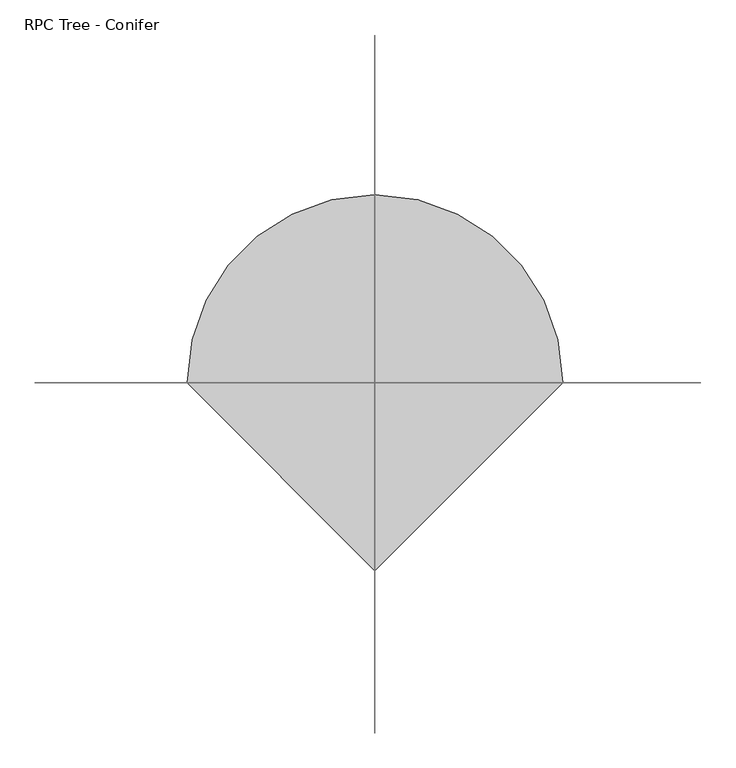
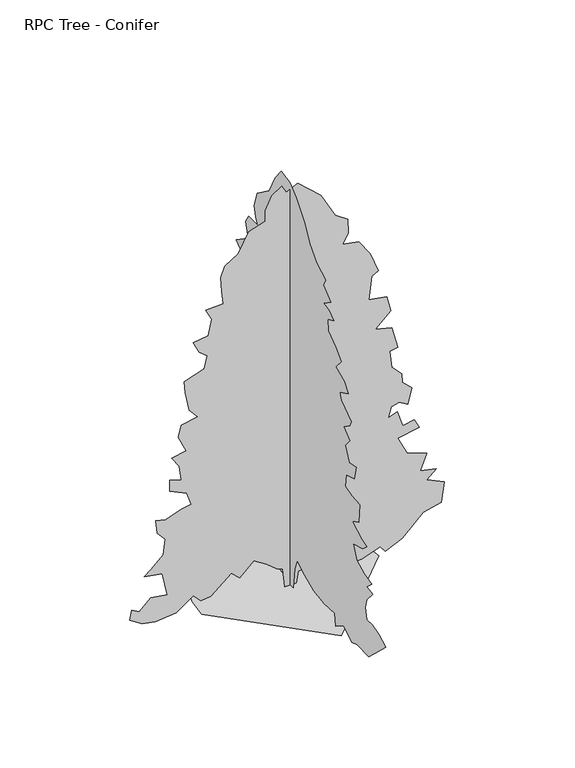
"""IFC4 building model written with IfcOpenShell, lengths in millimetres: geographic element geometry, RPC Tree - Conifer : Colorado Spruce - 13'."""

from ifc_helpers import new_model, si_unit, origin, place, context, project, spatial, triangles, source, transform, mapped, element, save


def rpc_tree_conifer_d3253eb6(model_context):
    return source(origin(), model_context, "Body", "Tessellation", [
        triangles([(0.1966733, -49.3561489, 3.58e-05), (0.1966807, -76.1744156, 207.8417467), (0.196685, -109.6973104, 301.7045676), (0.1966884, -230.379379, 234.6600225), (0.1966932, -377.8792239, 174.3188474), (0.1966999, -545.4937022, 147.5005898), (0.1967076, -713.5737408, 154.6348927), (0.196705, -733.2223234, 40.2275228), (0.1967129, -853.9046373, 120.682323), (0.196716, -981.9569956, 35.9934516), (0.1967211, -1075.1551586, 67.0457895), (0.196729, -1256.1798649, 60.3411615), (0.1967353, -1343.3377716, 140.7959572), (0.1967491, -1531.0664291, 321.8186923), (0.1967456, -1417.0879211, 375.4547353), (0.1967421, -1316.5197865, 408.9791061), (0.1967377, -1222.8412022, 401.1533847), (0.19674, -1202.5413511, 509.5473135), (0.196744, -1229.359409, 603.4116059), (0.1967514, -1323.2237377, 710.6836555), (0.1967478, -1229.359409, 730.7978348), (0.1967531, -1303.1095585, 797.8441057), (0.196749, -1189.1335939, 831.3659695), (0.1967454, -1068.45128, 891.7084345), (0.1967463, -1006.4049946, 1015.8652456), (0.1967546, -1162.3155361, 1059.3228401), (0.1967594, -1229.359409, 1119.6627617), (0.1967561, -1142.2014296, 1139.7769409), (0.1967521, -994.7010578, 1226.9373184), (0.1967585, -1101.9731438, 1280.5734341), (0.1967642, -1110.6508118, 1457.1305351), (0.1967592, -987.9947084, 1475.0058975), (0.1967552, -880.7226225, 1501.8238827), (0.1967595, -896.547456, 1623.9847401), (0.1967665, -1027.1927519, 1660.8127247), (0.1967716, -1055.0409794, 1790.1206749), (0.1967662, -947.7689661, 1770.0064957), (0.1967671, -880.024264, 1900.4932983), (0.1967731, -954.4728447, 1991.2570896), (0.1967713, -860.6085159, 2071.7111904), (0.1967775, -954.4728447, 2138.7573887), (0.1967803, -981.2908298, 2192.3935043), (0.196776, -813.6763515, 2299.6680611), (0.1967771, -793.562245, 2366.7117886), (0.1967851, -927.6547869, 2433.7581322), (0.196785, -867.3123945, 2520.9283928), (0.1967808, -733.2223234, 2581.2558151), (0.1967877, -820.3802301, 2681.8267113), (0.1967861, -726.515974, 2768.9745895), (0.1967833, -605.8360946, 2856.1474663), (0.1967862, -599.1297452, 2963.42929), (0.1967921, -699.6979162, 3010.3589836), (0.1967904, -625.9502375, 3064.0001862), (0.1967871, -538.7898236, 3084.1091331), (0.1967946, -652.7682226, 3164.5460838), (0.196792, -532.085945, 3258.4301788), (0.1967955, -565.6078451, 3325.4691101), (0.1967916, -424.8113883, 3405.9304779), (0.1967901, -310.832953, 3526.610321), (0.1967913, -235.627587, 3681.4162788), (0.1967901, -96.2880544, 3848.4313751), (0.1967879, 10.9852091, 3935.5795441), (0.1967827, 145.0765916, 3962.4), (0.1967749, 238.9406479, 3841.7201569), (0.1967651, 332.804468, 3654.0013824), (0.1967522, 527.2369314, 3513.1875938), (0.1967452, 580.8729744, 3359.0007843), (0.1967436, 554.0549529, 3265.1166893), (0.1967433, 520.5330528, 3204.7889763), (0.1967367, 668.0334246, 3204.7889763), (0.1967322, 714.9655163, 3124.3276085), (0.1967298, 674.7373032, 2983.5385277), (0.1967176, 862.465888, 2856.1474663), (0.1967187, 802.1234957, 2802.5065544), (0.1967143, 835.6479029, 2701.9356583), (0.1967057, 942.9199162, 2574.5445969), (0.1967072, 795.4196171, 2406.9400017), (0.1966989, 950.7208935, 2358.4253757), (0.1966939, 1036.7842449, 2319.782095), (0.1966878, 976.4418526, 2024.779026), (0.1966811, 1077.0125307, 1951.0287312), (0.1966784, 1056.8983515, 1830.3464172), (0.1966807, 929.5096882, 1716.3705254), (0.1966693, 1103.8305159, 1595.6882114), (0.1966656, 1003.2623085, 1320.7991764), (0.1966582, 1150.7626802, 1293.9811913), (0.1966531, 1224.5129025, 1233.6412697), (0.1966553, 1077.0125307, 1086.1408979), (0.1966461, 1264.7386448, 1059.3228401), (0.1966425, 1197.6948446, 838.0699207), (0.196648, 1016.6701384, 750.9119413), (0.1966429, 1077.0125307, 670.4579132), (0.1966358, 1217.8064804, 643.6398554), (0.1966273, 1304.9668579, 489.4331706), (0.1966198, 1418.9453659, 408.9791061), (0.1966101, 1519.5135006, 234.6600225), (0.1966177, 1304.9668579, 167.614224), (0.1966245, 1173.3830292, 197.6893322), (0.1966363, 887.0773218, 162.532194), (0.1966489, 580.8729744, 127.3867012), (0.1966585, 419.962411, 207.8417467), (0.1966599, 352.9185745, 154.204977), (0.1966604, 292.5761822, 80.4548002), (0.1966666, 131.6673356, 46.9321508), (0.1966712, 85.0868485, 132.0635687), (0.1966685, 57.9171634, 3.26e-05), (-50.7214044, -1.3e-06, 3.59e-05), (-70.8350431, 2.06e-05, 181.023489), (-124.4715721, 1.99e-05, 201.1371233), (-218.3356374, 2.07e-05, 281.5929136), (-339.0169521, 2.04e-05, 355.3430632), (-466.4056518, -3.2e-06, 234.6600225), (-546.8596799, -2.3e-06, 308.4109351), (-734.5883011, -1.51e-05, 147.5005898), (-828.8563116, -1.84e-05, 135.7027906), (-895.49643, -1.72e-05, 207.8417467), (-1056.4070297, -2.68e-05, 100.5686797), (-1250.8394932, -4.79e-05, 80.4550455), (-1371.5218071, -5.06e-05, 100.5686797), (-1485.5003151, -5.07e-05, 174.3188474), (-1465.3861359, -4.59e-05, 268.1826675), (-1398.3397923, -4.57e-05, 227.9553809), (-1291.0653809, -2.36e-05, 328.525078), (-1136.8610579, -2.02e-05, 301.7045676), (-1182.3370611, -1.16e-05, 523.1482275), (-1351.4077732, -1.52e-05, 556.4794415), (-1291.0653809, -1.13e-05, 603.4116059), (-1177.0893436, -3.1e-06, 710.6836555), (-1156.9752371, 3.8e-06, 851.4801487), (-1230.7254593, 5.5e-06, 938.6405262), (-1244.1356873, 1.08e-05, 1066.0267914), (-1150.2713585, 1.24e-05, 1039.2087336), (-1009.4748653, 3.34e-05, 1092.8447765), (-915.6106092, 3.71e-05, 1112.9588831), (-955.8388224, 4.13e-05, 1233.6412697), (-1116.8906199, 3.98e-05, 1309.0705318), (-1116.7469513, 4.46e-05, 1414.6635052), (-1009.4748653, 4.63e-05, 1381.1415688), (-1027.5656942, 5.21e-05, 1523.6492947), (-1096.6353155, 5.44e-05, 1622.5061966), (-962.542701, 5.96e-05, 1649.3241817), (-1036.2929232, 6.46e-05, 1810.2323833), (-1009.4748653, 7.02e-05, 1917.5069401), (-855.2706877, 9.04e-05, 1944.3249252), (-935.7247158, 9.22e-05, 2038.189254), (-969.2465796, 9.93e-05, 2219.2114895), (-982.6568802, 0.000104, 2333.1898521), (-794.9282227, 0.0001123, 2393.5297737), (-768.1102375, 0.0001185, 2514.2171745), (-841.860387, 0.000119, 2574.5445969), (-895.49643, 0.0001222, 2681.8267113), (-759.157659, 0.0001417, 2704.7837402), (-727.8819517, 0.0001494, 2856.1474663), (-781.5179947, 0.0001526, 2963.42929), (-620.6098658, 0.0001577, 2970.1160912), (-634.0176956, 0.0001629, 3097.5071526), (-640.724045, 0.0001687, 3231.6097229), (-607.1996015, 0.0001742, 3332.1803284), (-482.926373, 0.0001957, 3408.5803162), (-385.9491165, 0.0002069, 3593.6492523), (-231.7446482, 0.0002136, 3640.5789459), (-231.7446482, 0.0002181, 3741.1495514), (-171.4034912, 0.0002256, 3868.5406128), (-77.5396711, 0.0002311, 3928.8683258), (-37.3121507, 0.000229, 3855.1178856), (69.9609141, 0.000249, 3908.7590881), (284.5062896, 0.0002467, 3714.3290955), (418.5988678, 0.0002255, 3472.9694092), (532.5773031, 0.0002397, 3392.5077507), (539.2812181, 0.0002195, 3258.4301788), (485.6451751, 0.0002137, 3164.5460838), (633.1454378, 0.0002169, 3137.7503357), (740.4175238, 0.0002132, 2983.5385277), (814.167746, 0.0002067, 2789.108535), (753.1764833, 0.0002035, 2757.3845993), (727.0097666, 0.0001927, 2534.3264122), (894.6217741, 0.0001965, 2507.5056656), (928.1461813, 0.0001909, 2360.0079826), (787.3496881, 0.0001807, 2225.9177662), (941.5539385, 0.0001835, 2185.6895531), (995.1924522, 0.0001614, 1977.8468616), (921.4397593, 0.0001587, 1964.4391045), (941.5539385, 0.0001521, 1803.5284321), (1030.220038, 0.0001504, 1706.6750416), (1035.4181946, 0.0001468, 1622.5061966), (1122.5786448, 0.0001455, 1535.3458191), (1089.0542376, 0.0001379, 1387.84552), (1008.6002094, 0.0001376, 1434.7775391), (934.8500599, 0.0001345, 1414.6635052), (908.0320021, 0.0001295, 1320.7991764), (988.4861029, 0.0001331, 1347.6171616), (1042.1220732, 0.0001278, 1193.4129839), (1149.3966299, 0.0001319, 1213.5270905), (1196.3287943, 0.0001294, 1126.366713), (995.1924522, 0.0001216, 1086.1408979), (1082.350359, 0.000102, 911.8200703), (1263.3750652, 0.0001188, 844.7762701), (1205.4472784, 9.61e-05, 697.2783691), (1350.532972, 9.89e-05, 663.7515638), (1263.3750652, 9.3e-05, 590.001378), (1424.2832668, 9.42e-05, 509.5473135), (1397.4651363, 8.5e-05, 321.8186923), (1229.850658, 7.82e-05, 281.5929136), (1036.3395046, 6.4e-05, 93.3593451), (881.2140169, 4.18e-05, 20.1136387), (834.2818525, 4.31e-05, 80.4548002), (658.291868, 3.51e-05, 20.7551739), (472.2349108, 2.93e-05, 13.4091084), (398.4847612, 3.01e-05, 80.4548002), (230.8705009, 2.78e-05, 140.7959572), (72.6778858, 2.16e-05, 108.3902136), (56.5516581, 1.63e-05, 3.27e-05), (-820.443671, 4.5e-06, 5.88e-05), (-798.7470303, 188.0361787, 5.26e-05), (-736.9608307, 360.7170811, 4.56e-05), (-640.0281572, 513.0961158, 3.82e-05), (-512.8994345, 640.2248022, 3.06e-05), (-360.5203998, 737.1574757, 2.32e-05), (-187.8395156, 798.9436752, 1.62e-05), (0.1967069, 820.640316, 9.9e-06), (188.2328419, 798.9436752, 5e-06), (360.9137624, 737.1574757, 1.7e-06), (513.2927971, 640.2248022, 0.0), (640.4214472, 513.0961158, 0.0), (737.3541206, 360.7170811, 1.7e-06), (799.1403202, 188.0361787, 5e-06), (820.836961, -7.6e-05, 9.9e-06), (0.1965635, -820.640316, 5.88e-05)], [[27, 26, 28], [22, 21, 23], [20, 19, 21], [52, 51, 53], [8, 7, 9], [36, 35, 37], [14, 13, 15], [35, 34, 37], [55, 54, 56], [73, 72, 74], [96, 95, 97], [89, 88, 90], [45, 44, 46], [87, 86, 88], [86, 85, 88], [53, 51, 54], [46, 44, 47], [90, 88, 91], [15, 13, 16], [16, 13, 17], [39, 38, 40], [26, 25, 28], [28, 25, 29], [48, 47, 49], [57, 56, 58], [31, 30, 32], [30, 29, 32], [42, 41, 43], [41, 40, 43], [1, 106, 2], [106, 105, 2], [76, 75, 77], [95, 94, 97], [97, 94, 98], [79, 78, 80], [84, 83, 85], [32, 29, 33], [104, 103, 105], [13, 12, 17], [12, 11, 17], [78, 77, 80], [103, 102, 105], [63, 62, 64], [81, 80, 82], [82, 80, 83], [62, 61, 64], [64, 61, 65], [61, 60, 65], [60, 59, 65], [70, 69, 71], [71, 69, 72], [98, 94, 99], [94, 93, 99], [93, 92, 99], [99, 92, 100], [92, 91, 100], [100, 91, 101], [49, 47, 50], [10, 9, 11], [11, 9, 17], [17, 9, 18], [9, 7, 18], [65, 59, 66], [66, 59, 67], [67, 59, 68], [68, 59, 69], [59, 58, 69], [58, 56, 69], [56, 54, 69], [69, 54, 72], [54, 51, 72], [51, 50, 72], [72, 50, 74], [74, 50, 75], [75, 50, 77], [50, 47, 77], [47, 44, 77], [44, 43, 77], [43, 40, 77], [77, 40, 80], [80, 40, 83], [40, 38, 83], [83, 38, 85], [38, 37, 85], [37, 34, 85], [34, 33, 85], [33, 29, 85], [29, 25, 85], [85, 25, 88], [88, 25, 91], [91, 25, 101], [101, 25, 102], [25, 24, 102], [24, 23, 102], [23, 21, 102], [2, 105, 3], [105, 102, 3], [102, 21, 3], [3, 21, 4], [4, 21, 5], [5, 21, 6], [6, 21, 7], [7, 21, 18], [21, 19, 18], [126, 125, 127], [199, 198, 200], [154, 153, 155], [140, 139, 141], [131, 130, 132], [121, 120, 122], [120, 119, 122], [187, 186, 188], [137, 136, 138], [136, 135, 138], [151, 150, 152], [194, 193, 195], [193, 192, 195], [127, 125, 128], [181, 180, 182], [164, 163, 165], [186, 185, 188], [197, 196, 198], [191, 190, 192], [112, 111, 113], [107, 212, 108], [212, 211, 108], [174, 173, 175], [150, 149, 152], [180, 179, 182], [130, 129, 132], [147, 146, 148], [205, 204, 206], [201, 200, 202], [202, 200, 203], [163, 162, 165], [192, 190, 195], [166, 165, 167], [119, 118, 122], [122, 118, 123], [123, 118, 124], [118, 117, 124], [117, 116, 124], [177, 176, 178], [178, 176, 179], [132, 129, 133], [188, 185, 189], [143, 142, 144], [142, 141, 144], [162, 161, 165], [165, 161, 167], [167, 161, 168], [124, 116, 125], [146, 145, 148], [145, 144, 148], [115, 114, 116], [114, 113, 116], [116, 113, 125], [125, 113, 128], [128, 113, 129], [129, 113, 133], [133, 113, 134], [113, 111, 134], [169, 168, 170], [170, 168, 171], [168, 161, 171], [161, 160, 171], [160, 159, 171], [159, 158, 171], [158, 157, 171], [157, 156, 171], [156, 155, 171], [172, 171, 173], [173, 171, 175], [171, 155, 175], [175, 155, 176], [155, 153, 176], [153, 152, 176], [152, 149, 176], [176, 149, 179], [149, 148, 179], [148, 144, 179], [179, 144, 182], [182, 144, 183], [144, 141, 183], [141, 139, 183], [139, 138, 183], [138, 135, 183], [135, 134, 183], [134, 111, 183], [111, 110, 183], [183, 110, 184], [184, 110, 185], [185, 110, 189], [189, 110, 190], [190, 110, 195], [110, 109, 195], [109, 108, 195], [108, 211, 195], [211, 210, 195], [195, 210, 196], [210, 209, 196], [196, 209, 198], [209, 208, 198], [208, 207, 198], [207, 206, 198], [206, 204, 198], [204, 203, 198], [203, 200, 198], [228, 227, 213], [227, 226, 213], [213, 226, 214], [226, 225, 214], [214, 225, 215], [215, 225, 216], [225, 224, 216], [224, 223, 216], [216, 223, 217], [217, 223, 218], [218, 223, 219], [219, 223, 220], [220, 223, 221], [221, 223, 222]], closed=False),
    ])


if __name__ == "__main__":
    model = new_model("IFC4")
    model_context = context("Model", 3, world=origin())
    ifc_project = project(units=[si_unit("LENGTHUNIT", "METRE", prefix="MILLI")], contexts=[model_context])
    site = spatial("IfcSite", under=ifc_project)
    building = spatial("IfcBuilding", under=site)
    placement = place(None, origin())
    rpc_tree_conifer_shape = rpc_tree_conifer_d3253eb6(model_context)
    element("IfcGeographicElement", 1, ObjectType="RPC Tree - Conifer : Colorado Spruce - 13'", at=placement, inside=building, context=model_context, shape_type="MappedRepresentation", body=[
        mapped(rpc_tree_conifer_shape, transform((0.0, 0.0, 0.0), x_axis=(1.0, 0.0, 0.0), y_axis=(0.0, 1.0, 0.0), z_axis=(0.0, 0.0, 1.0))),
    ])
    save(model, "model.ifc")

# Revit data of these elements
# Type "RPC Tree - Conifer : Colorado Spruce - 13'"
#   built-in parameter 1005198 = "{2, 15},{39, RPC-16-G0M4-N9PX-U6TN-C000-ST1L-LVER-AU},{1, 0},{1, 0},{2, 35},{1, 8},{5, Color},{1, 0},{1, 0},{3, 0.8},{3, 0.8},{3, 0.8},{1, 8},{7, BBoxMin},{1, 0},{1, 0},{1, 0},{1, 0},{1, 0},{1, 8},{7, BBoxMax},{1, 0},{1, 0},{1, 0},{1, 0},{1, 0},{2, 11},{9, RPCTypeId},{1, 0},{1, 0},{39, RPC-16-G0M4-N9PX-U6TN-C000-ST1L-LVER-AU},{1, 6},{14, RPCPlantHeight},{1, 0},{1, 0},{2, 13},{2, 11},{7, keyword},{1, 0},{1, 0},{91, :Geometry:RPC:Colorado Spruce:colorado spruce:pinaceae:picea:pungens:evergreen:conifer:blue},{2, 11},{8, category},{1, 0},{1, 0},{16, :Trees [General]},{2, 11},{12, LocalizedUID},{1, 0},{1, 0},{15, Colorado Spruce},{2, 14},{6, Height},{1, 0},{1, 0},{2, 13},{1, 2},{16, Cast Reflections},{1, 0},{1, 0},{1, 0},{1, 2},{12, Cast Shadows},{1, 0},{1, 0},{1, 1},{1, 2},{9, Lock View},{1, 0},{1, 0},{1, 0},{1, 4},{5, ViewC},{1, 0},{1, 0},{1, 0},{2, 11},{20, AdvancedUIDefinition},{1, 0},{1, 0},{0, },{2, 11},{10, AssetLibID},{1, 0},{1, 0},{36, 4D3F6E72-3F99-4203-98E9-AF80B3C7A7A4},{2, 11},{10, BaseSchema},{1, 0},{1, 0},{9, RPCSchema},{2, 11},{12, ExchangeGUID},{1, 0},{1, 0},{0, },{1, 2},{6, Hidden},{1, 0},{1, 0},{1, 0},{1, 4},{11, RPCCategory},{1, 0},{1, 0},{1, 0},{2, 11},{8, RPCImage},{1, 0},{1, 0},{0, },{1, 4},{13, SchemaVersion},{1, 0},{1, 0},{1, 4},{2, 11},{12, UIDefinition},{1, 0},{1, 0},{0, },{2, 11},{6, UIName},{1, 0},{1, 0},{39, RPC-16-G0M4-N9PX-U6TN-C000-ST1L-LVER-AU},{2, 11},{11, VersionGUID},{1, 0},{1, 0},{9, RPCSchema},{2, 11},{9, assettype},{1, 0},{1, 0},{11, RPCGeometry},{2, 11},{11, description},{1, 0},{1, 0},{0, },{2, 11},{9, localname},{1, 0},{1, 0},{3, RPC},{2, 11},{9, localtype},{1, 0},{1, 0},{3, RPC},{1, 4},{8, revision},{1, 0},{1, 0},{1, 1},{2, 11},{9, thumbnail},{1, 0},{1, 0},{0, },{1, 4},{7, version},{1, 0},{1, 0},{1, 1},{1, 2},{20, RPC_Cast Reflections},{1, 0},{1, 0},{1, 1},{1, 2},{16, RPC_Cast Shadows},{1, 0},{1, 0},{1, 1},{1, 2},{13, RPC_Lock View},{1, 0},{1, 0},{1, 0},{1, 4},{9, RPC_ViewC},{1, 0},{1, 0},{1, 0},{21, assetlibrary_base.fbx},{1, 5},"
#   built-in parameter 1005195 = "RPC-16-G0M4-N9PX-U6TN-C000-ST1L-LVER-AU"
#   Type Comments = "Colorado Spruce"
#   Assembly Code = "G2050500"
#   Height = 396.24 cm
#   Description = (empty or 0)
#   Default Elevation = 0
